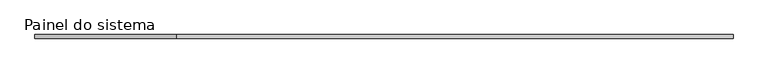
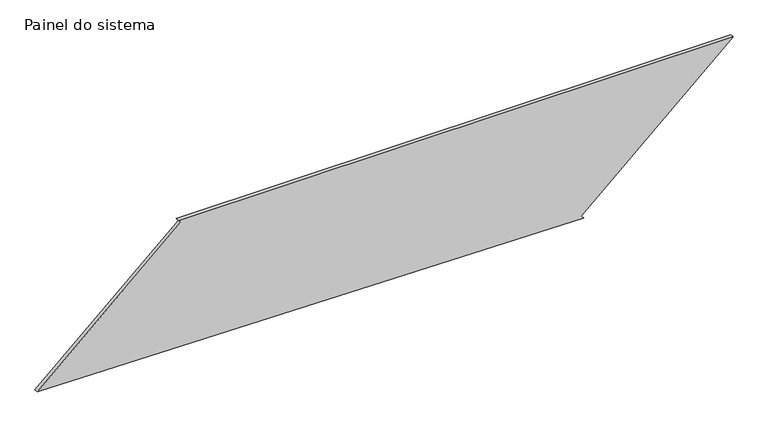
"""IFC4 building model written with IfcOpenShell, lengths in millimetres: plate geometry, Painel do sistema : Envidraçado."""

from ifc_helpers import new_model, si_unit, frame, origin, place, context, project, spatial, polyline, outline, extrude, source, transform, mapped, element, save


def painel_do_sistema_18c48899(model_context):
    return source(origin(), model_context, "Body", "SweptSolid", [
        extrude(outline(polyline([(0.0, 1364.7199669), (18.5968466, 1348.011966), (957.0073765, 2392.5101539), (957.0073765, -1419.479305), (938.4105299, -1402.7713041), (49.1975382, -2392.5101539), (0.0, 1364.7199669)])), frame((0.0, 24.5, 0.0), z_axis=(0.0, 1.0, 0.0), x_axis=(0.0, 0.0, 1.0)), (0.0, 0.0, 1.0), 25.0),
    ])


if __name__ == "__main__":
    model = new_model("IFC4")
    model_context = context("Model", 3, world=origin())
    ifc_project = project(units=[si_unit("LENGTHUNIT", "METRE", prefix="MILLI")], contexts=[model_context])
    site = spatial("IfcSite", under=ifc_project)
    building = spatial("IfcBuilding", under=site)
    placement = place(None, origin())
    painel_do_sistema_shape = painel_do_sistema_18c48899(model_context)
    element("IfcPlate", 1, ObjectType="Painel do sistema : Envidraçado", at=placement, inside=building, context=model_context, shape_type="MappedRepresentation", body=[
        mapped(painel_do_sistema_shape, transform((0.0, 0.0, 0.0), x_axis=(1.0, 0.0, 0.0), y_axis=(0.0, 1.0, 0.0), z_axis=(0.0, 0.0, 1.0))),
    ])
    save(model, "model.ifc")

# Revit data of these elements
# Type "Painel do sistema : Envidraçado"
#   Construction Type Id = "GSP4R"
#   Analytic Construction = "Vidraça única Pilkington 1/8 pol"
#   Visual Light Transmittance = 0.9
#   Solar Heat Gain Coefficient = 0.86
#   Heat Transfer Coefficient (U) = 6.7069 W/(m²·K)
# Element 1 (IfcPlate, "Painel do sistema : Envidraçado")
#   Materials on its faces: "Vidro"
# Materials
#   "Vidro": class "Vidro", colour RGB 0 128 192, transparency 0.9, Description = "Vidro de sílica", Cost = 0
